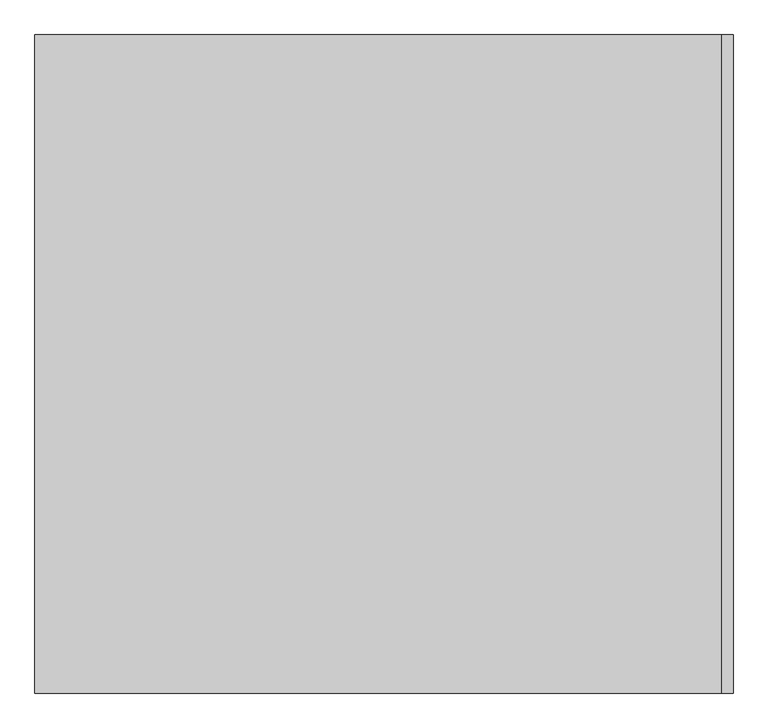
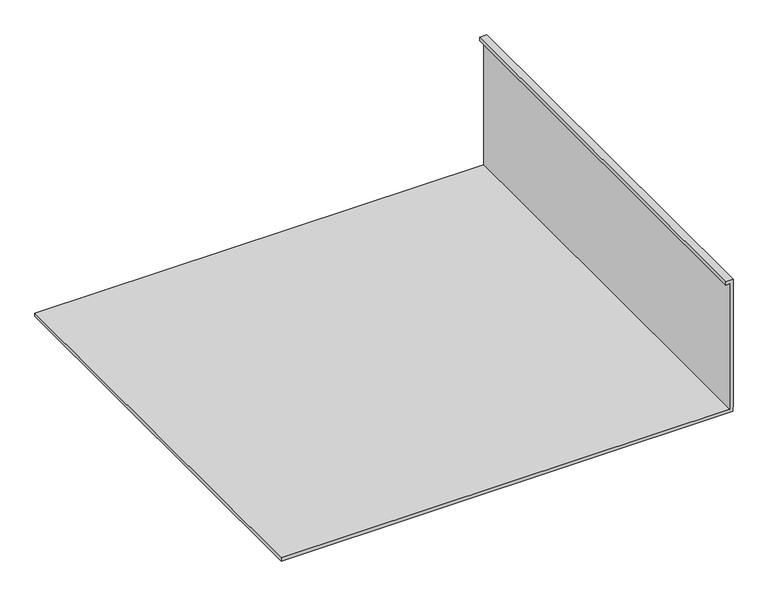
"""IFC4 building model written with IfcOpenShell, lengths in millimetres: proxy geometry, Gypsum022 10512 : Gypsum022 10512."""

from ifc_helpers import new_model, si_unit, frame, origin, place, context, project, spatial, polyline, outline, extrude, source, transform, mapped, element, save


def generic_models_a0bde621(model_context):
    return source(origin(), model_context, "Body", "SweptSolid", [
        extrude(outline(polyline([(42133.7076708, 4092.7965054), (42117.8326708, 4092.7965054), (42117.8326708, 6190.3055469), (42119.1126708, 6190.3055469), (42119.1126708, 6211.4587308), (42140.2658547, 6211.4587308), (42140.2658547, 6212.7387308), (42771.6902023, 6212.7387308), (42771.6902023, 6178.6060416), (42755.8152023, 6178.6060416), (42755.8152023, 6196.8637308), (42133.7076708, 6196.8637308), (42133.7076708, 4092.7965054)])), frame((0.0, -1052.8912332, 0.0), z_axis=(0.0, 1.0, 0.0), x_axis=(0.0, 0.0, 1.0)), (0.0, 0.0, 1.0), 1999.85),
    ])


if __name__ == "__main__":
    model = new_model("IFC4")
    model_context = context("Model", 3, world=origin())
    ifc_project = project(units=[si_unit("LENGTHUNIT", "METRE", prefix="MILLI")], contexts=[model_context])
    site = spatial("IfcSite", under=ifc_project)
    building = spatial("IfcBuilding", under=site)
    placement = place(None, origin())
    generic_models_shape = generic_models_a0bde621(model_context)
    element("IfcBuildingElementProxy", 1, Name="Gypsum022 10512 : Gypsum022 10512", ObjectType="Gypsum022 10512 : Gypsum022 10512", at=placement, inside=building, context=model_context, shape_type="MappedRepresentation", body=[
        mapped(generic_models_shape, transform((0.0, 0.0, 0.0), x_axis=(1.0, 0.0, 0.0), y_axis=(0.0, 1.0, 0.0), z_axis=(0.0, 0.0, 1.0))),
    ])
    save(model, "model.ifc")

# Revit data of these elements
# Type "Gypsum022 10512 : Gypsum022 10512"
#   NameOverride = "Gypsum022"
# Element 1 (IfcBuildingElementProxy, "Gypsum022 10512 : Gypsum022 10512")
#   Materials on its faces: "5/8\" GYPSUM BOARD"
# Materials
#   "5/8\" GYPSUM BOARD": class "Unassigned", colour RGB 214 214 214, transparency 0, Cost = 0
